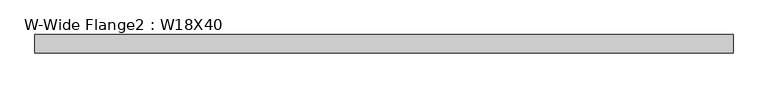
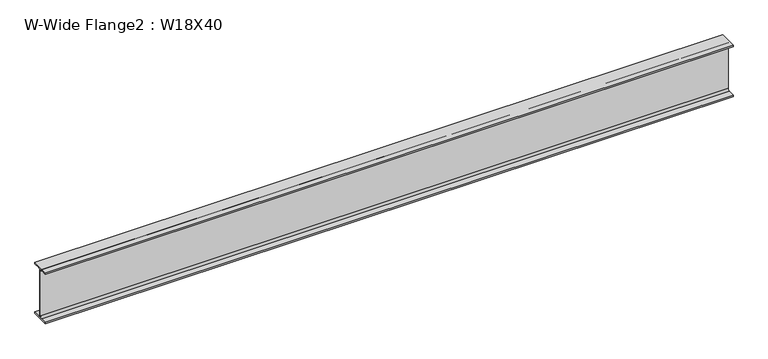
"""IFC4 building model written with IfcOpenShell, lengths in millimetres: beam geometry, W-Wide Flange2 : W18X40."""

from ifc_helpers import new_model, si_unit, point, frame, frame_2d, origin, place, context, project, spatial, polyline, circle_curve, trimmed, segment, composite_curve, outline, extrude, source, transform, mapped, element, save


def w_wide_flange2_w18x40_ca46fc5e(model_context):
    return source(origin(), model_context, "Body", "SweptSolid", [
        extrude(outline(composite_curve([segment(polyline([(76.454, -213.995), (76.454, -227.33), (-76.454, -227.33), (-76.454, -213.995), (-20.828, -213.995)]), True, "CONTINUOUS"), segment(trimmed(circle_curve(frame_2d((-20.828, -197.1675)), 16.8275), [point((-20.828, -213.995))], [point((-4.0005, -197.1675))], True, "CARTESIAN"), True, "CONTINUOUS"), segment(polyline([(-4.0005, -197.1675), (-4.0005, 197.1675)]), True, "CONTINUOUS"), segment(trimmed(circle_curve(frame_2d((-20.828, 197.1675)), 16.8275), [point((-4.0005, 197.1675))], [point((-20.828, 213.995))], True, "CARTESIAN"), True, "CONTINUOUS"), segment(polyline([(-20.828, 213.995), (-76.454, 213.995), (-76.454, 227.33), (76.454, 227.33), (76.454, 213.995), (20.828, 213.995)]), True, "CONTINUOUS"), segment(trimmed(circle_curve(frame_2d((20.828, 197.1675)), 16.8275), [point((20.828, 213.995))], [point((4.0005, 197.1675))], True, "CARTESIAN"), True, "CONTINUOUS"), segment(polyline([(4.0005, 197.1675), (4.0005, -197.1675)]), True, "CONTINUOUS"), segment(trimmed(circle_curve(frame_2d((20.828, -197.1675)), 16.8275), [point((4.0005, -197.1675))], [point((20.828, -213.995))], True, "CARTESIAN"), True, "CONTINUOUS"), segment(polyline([(20.828, -213.995), (76.454, -213.995)]), True, "CONTINUOUS")], self_intersect=False)), frame((-2876.153125, 0.0, 0.0), z_axis=(1.0, 0.0, 0.0), x_axis=(0.0, 1.0, 0.0)), (0.0, 0.0, 1.0), 5757.465625),
    ])


if __name__ == "__main__":
    model = new_model("IFC4")
    model_context = context("Model", 3, world=origin())
    ifc_project = project(units=[si_unit("LENGTHUNIT", "METRE", prefix="MILLI")], contexts=[model_context])
    site = spatial("IfcSite", under=ifc_project)
    building = spatial("IfcBuilding", under=site)
    placement = place(None, origin())
    w_wide_flange2_w18x40_shape = w_wide_flange2_w18x40_ca46fc5e(model_context)
    element("IfcBeam", 1, ObjectType="W-Wide Flange2 : W18X40", at=placement, inside=building, context=model_context, shape_type="MappedRepresentation", body=[
        mapped(w_wide_flange2_w18x40_shape, transform((0.0, 0.0, 0.0), x_axis=(1.0, 0.0, 0.0), y_axis=(0.0, 1.0, 0.0), z_axis=(0.0, 0.0, 1.0))),
    ])
    save(model, "model.ifc")

# Revit data of these elements
# Type "W-Wide Flange2 : W18X40"
#   Assembly Code = "B10"
#   W = 40
#   Length [instance default] = 5' - 0"
#   bf = 0' - 6.02"
#   d = 1' - 5.9"
#   k = 0' - 1 3/16"
#   k2 = 0' - 0.6625"
#   tf = 0' - 0.525"
#   tw = 0' - 0.315"
#   A = 0.0819444 SF
#   Structural Material [instance default] = Steel ASTM A992
# Element 1 (IfcBeam, "W-Wide Flange2 : W18X40")
#   Materials on its faces: "Steel ASTM A992"
# Materials
#   "Steel ASTM A992": class "Metal", colour RGB 199 199 199, transparency 0, Description = "Structural steel 50ksi", Cost = 0
